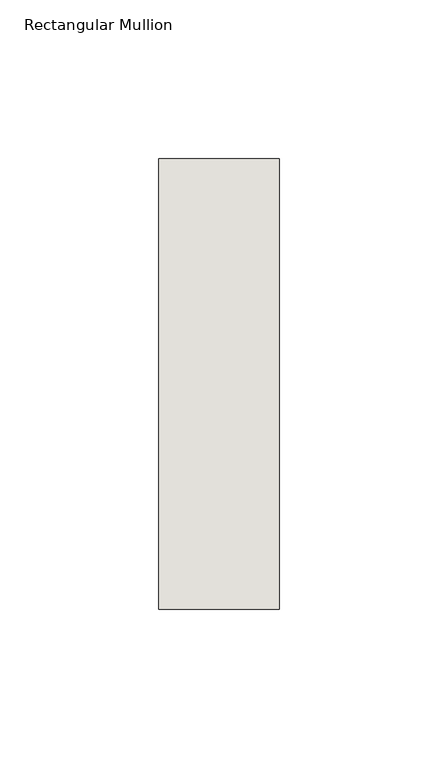
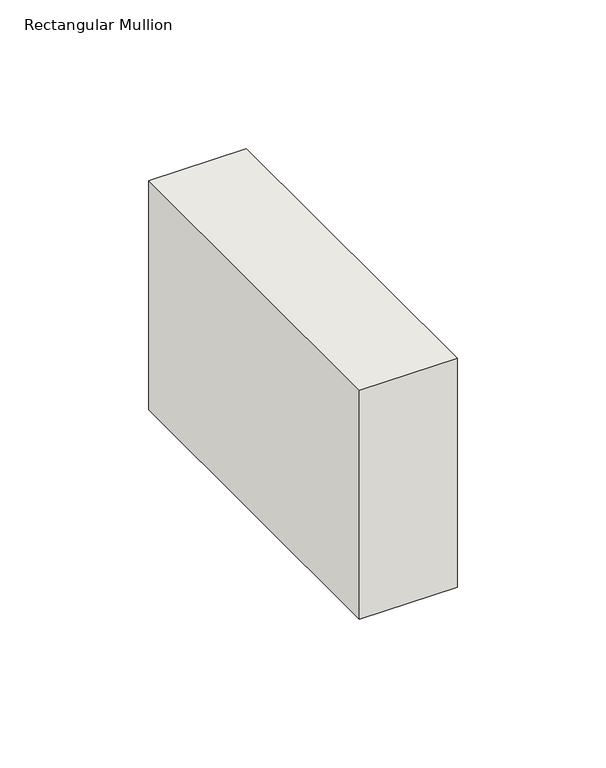
"""IFC4 building model written with IfcOpenShell, lengths in millimetres: wall geometry, Rectangular Mullion : NLRS_21_CWM_hsb-regel 38x142_gen_rsf."""

from ifc_helpers import new_model, si_unit, frame, origin, place, context, project, spatial, polyline, outline, extrude, source, transform, mapped, element, save


def rectangular_mullion_b209e97a(model_context):
    return source(origin(), model_context, "Body", "SweptSolid", [
        extrude(outline(polyline([(-38.0, -71.0), (-38.0, 71.0), (0.0, 71.0), (0.0, -71.0), (-38.0, -71.0)])), frame((0.0, 0.0, -94.1558939), z_axis=(0.0, 0.0, 1.0), x_axis=(1.0, 0.0, 0.0)), (0.0, 0.0, 1.0), 94.1558939),
    ])


if __name__ == "__main__":
    model = new_model("IFC4")
    model_context = context("Model", 3, world=origin())
    ifc_project = project(units=[si_unit("LENGTHUNIT", "METRE", prefix="MILLI")], contexts=[model_context])
    site = spatial("IfcSite", under=ifc_project)
    building = spatial("IfcBuilding", under=site)
    placement = place(None, origin())
    rectangular_mullion_shape = rectangular_mullion_b209e97a(model_context)
    element("IfcWall", 1, ObjectType="Rectangular Mullion : NLRS_21_CWM_hsb-regel 38x142_gen_rsf", at=placement, inside=building, context=model_context, shape_type="MappedRepresentation", body=[
        mapped(rectangular_mullion_shape, transform((0.0, 0.0, 0.0), x_axis=(1.0, 0.0, 0.0), y_axis=(0.0, 1.0, 0.0), z_axis=(0.0, 0.0, 1.0))),
    ])
    save(model, "model.ifc")

# Revit data of these elements
# Type "Rectangular Mullion : NLRS_21_CWM_hsb-regel 38x142_gen_rsf"
#   Type IfcGUID = "07M7mRoiH1CR8m_RSKIwpF"
#   Assembly Code = "21.10"
#   IfcExportAs = "IfcWall"
#   built-in parameter 1007322 = 0.465879 (stored number, unit not read)
#   built-in parameter 1007321 = 0.062336 (stored number, unit not read)
#   built-in parameter 1007320 = 0.062336 (stored number, unit not read)
# Element 1 (IfcWall, "Rectangular Mullion : NLRS_21_CWM_hsb-regel 38x142_gen_rsf")
#   Materials on its faces: "NLRS_i2_hout naaldhout vuren_gen_rsf"
# Materials
#   "NLRS_i2_hout naaldhout vuren_gen_rsf": class "I - Hout", colour RGB 234 199 147, transparency 0, Keynote = "i2", Manufacturer = "Revit Standards Foundation", URL = "www.revitstandards.org", Description = "hout vuren", Cost = 0
